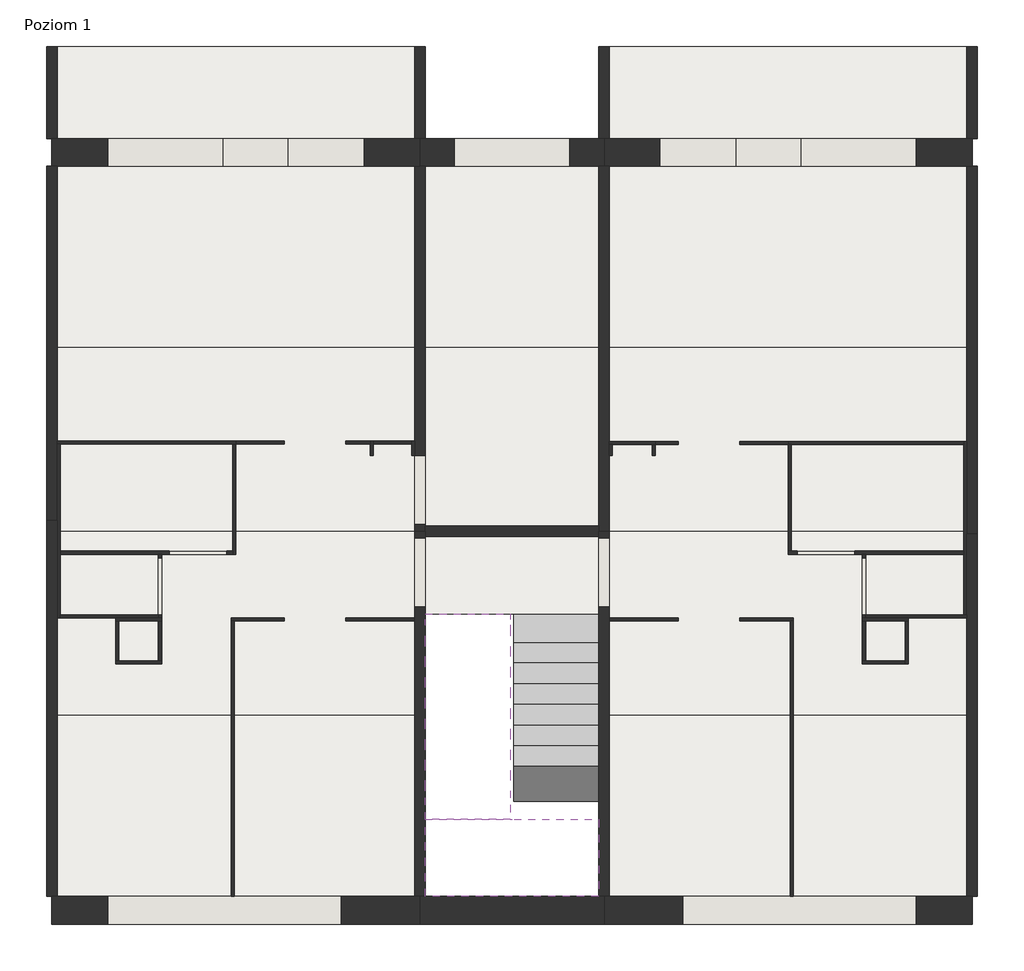
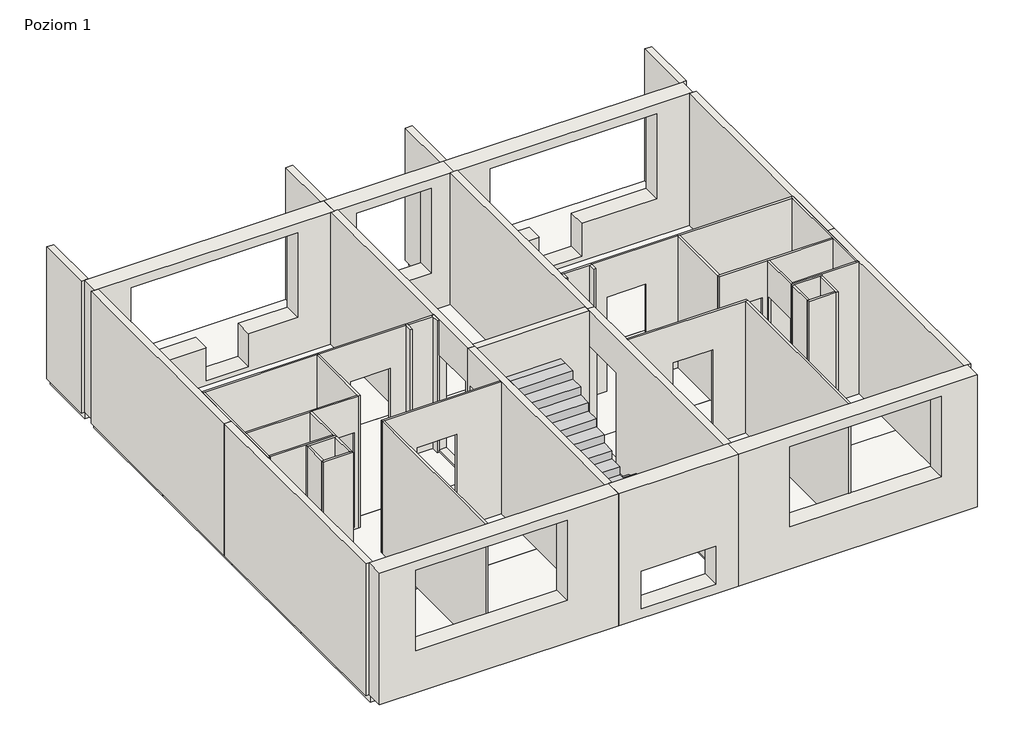
# One storey: 51 walls, 14 slabs, 2 proxies.
# Revit data of these elements (continued)
# Element 19 (IfcWall, "Prefab_ext_wall") (continued)
#   LastInspectionDate = 2025
#   MaintenanceInterval = 30
#   Phase Created = Etap 1
#   Base Constraint = Poziom 1
#   Top Constraint = Poziom 2
#   Materials on its faces: "Beton, wylewany na miejscu budowy"
# Element 20 (IfcWall, "Prefab_ext_wall")
#   CircularElementName = "Prefabricated Exterior Loadbearing Reinforced Concrete Wall"
#   CircularElementlDescription = "Medium conditions, damage in lower part"
#   CircularityNotes = "With exterior window opening"
#   Top Offset = 0 mm
#   Base Offset = 0 mm
#   wall height = 2800 mm
#   ExpectedServiceLife = 50
#   InstallationYear = 1973
#   LastInspectionDate = 2025
#   MaintenanceInterval = 30
#   Phase Created = Etap 1
#   Base Constraint = Poziom 1
#   Top Constraint = Poziom 2
#   Materials on its faces: "Beton, wylewany na miejscu budowy"
# Element 21 (IfcWall, "Prefab_ext_wall")
#   CircularElementName = "Prefabricated Exterior Loadbearing Reinforced Concrete Wall"
#   CircularElementlDescription = "Good condition"
#   CircularityNotes = "With exterior window opening"
#   Top Offset = 0 mm
#   Base Offset = 0 mm
#   wall height = 2800 mm
#   ExpectedServiceLife = 50
#   InstallationYear = 1973
#   MaintenanceInterval = 30
#   Phase Created = Etap 1
#   Base Constraint = Poziom 1
#   Top Constraint = Poziom 2
#   Materials on its faces: "Beton, wylewany na miejscu budowy"
# Element 22 (IfcWall, "Prefab_ext_wall")
#   CircularElementName = "Prefabricated Exterior Loadbearing Reinforced Concrete Wall"
#   CircularElementlDescription = "Bad condition"
#   CircularityNotes = "With exterior window opening"
#   Top Offset = 0 mm
#   Base Offset = 0 mm
#   wall height = 2800 mm
#   ExpectedServiceLife = 50
#   InstallationYear = 1973
#   MaintenanceInterval = 30
#   Phase Created = Etap 1
#   Base Constraint = Poziom 1
#   Top Constraint = Poziom 2
#   Materials on its faces: "Beton, wylewany na miejscu budowy"
# Element 23 (IfcWall, "Prefab_int_wall")
#   CircularElementName = "Prefabricated Reinforced Reinforced Concrete Bathroom Wall"
#   CircularElementlDescription = "The element looks to be in medium condition, mold present"
#   Top Offset = 0 mm
#   Base Offset = 0 mm
#   wall height = 2800 mm
#   ExpectedServiceLife = 50
#   InstallationYear = 1973
#   LastInspectionDate = 2025
#   MaintenanceInterval = 20
#   Phase Created = Etap 1
#   Base Constraint = Poziom 1
#   Top Constraint = Poziom 2
#   Materials on its faces: "Beton, wylewany na miejscu budowy"
# Elements 24, 26 (IfcWall, "Prefab_int_wall")
#   CircularElementName = "Prefabricated Reinforced Reinforced Concrete Interior Wall"
#   CircularElementlDescription = "Good condition, no major damage"
#   CircularityNotes = "With door opening"
#   Top Offset = 0 mm
#   Base Offset = 0 mm
#   wall height = 2800 mm
#   ExpectedServiceLife = 50
#   InstallationYear = 1973
#   LastInspectionDate = 2025
#   MaintenanceInterval = 40
#   Phase Created = Etap 1
#   Base Constraint = Poziom 1
#   Top Constraint = Poziom 2
#   Materials on its faces: "Beton, wylewany na miejscu budowy"
# Element 25 (IfcWall, "Prefab_int_wall")
#   CircularElementName = "Prefabricated Reinforced Reinforced Concrete Interior Wall"
#   CircularElementlDescription = "The element looks to be in good condition, no major damage"
#   Top Offset = 0 mm
#   Base Offset = 0 mm
#   wall height = 2800 mm
#   ExpectedServiceLife = 50
#   InstallationYear = 1973
#   LastInspectionDate = 2025
#   MaintenanceInterval = 40
#   Phase Created = Etap 1
#   Base Constraint = Poziom 1
#   Top Constraint = Poziom 2
#   Materials on its faces: "Beton, wylewany na miejscu budowy"
# Element 27 (IfcWall, "Prefab_int_wall")
#   CircularElementName = "Prefabricated Reinforced Reinforced Concrete Interior Wall"
#   CircularElementlDescription = "Good condition, minor dents and holes"
#   Top Offset = 0 mm
#   Base Offset = 0 mm
#   wall height = 2800 mm
#   ExpectedServiceLife = 50
#   InstallationYear = 1973
#   LastInspectionDate = 2025
#   MaintenanceInterval = 40
#   Phase Created = Etap 1
#   Base Constraint = Poziom 1
#   Top Constraint = Poziom 2
#   Materials on its faces: "Beton, wylewany na miejscu budowy"
# Elements 28, 30, 32 (IfcWall, "Prefab_int_wall")
#   CircularElementName = "Prefabricated Reinforced Reinforced Concrete Shaft Wall"
#   Top Offset = 0 mm
#   Base Offset = 0 mm
#   wall height = 2800 mm
#   ExpectedServiceLife = 50
#   InstallationYear = 1973
#   LastInspectionDate = 2004
#   MaintenanceInterval = 40
#   Phase Created = Etap 1
#   Base Constraint = Poziom 1
#   Top Constraint = Poziom 2
#   Materials on its faces: "Beton, wylewany na miejscu budowy"
# Element 29 (IfcWall, "Prefab_int_wall")
#   CircularElementName = "Prefabricated Reinforced Reinforced Concrete Shaft Wall"
#   CircularElementlDescription = "The element looks to be in good condition, no major damage"
#   Top Offset = 0 mm
#   Base Offset = 0 mm
#   wall height = 2800 mm
#   ExpectedServiceLife = 50
#   InstallationYear = 1973
#   LastInspectionDate = 2004
#   MaintenanceInterval = 40
#   Phase Created = Etap 1
#   Base Constraint = Poziom 1
#   Top Constraint = Poziom 2
#   Materials on its faces: "Beton, wylewany na miejscu budowy"
# Element 31 (IfcWall, "Prefab_int_wall")
#   CircularElementName = "Prefabricated Reinforced Reinforced Concrete Bathroom Wall"
#   CircularElementlDescription = "Good condition, no major damage"
#   CircularityNotes = "With door opening"
#   Top Offset = 0 mm
#   Base Offset = 0 mm
#   wall height = 2800 mm
#   ExpectedServiceLife = 50
#   InstallationYear = 1973
#   LastInspectionDate = 2004
#   MaintenanceInterval = 20
#   Phase Created = Etap 1
#   Base Constraint = Poziom 1
#   Top Constraint = Poziom 2
#   Materials on its faces: "Beton, wylewany na miejscu budowy"
# Element 33 (IfcWall, "Prefab_int_wall")
#   CircularElementName = "Prefabricated Reinforced Reinforced Concrete Bathroom Wall"
#   CircularElementlDescription = "The element looks to be in medium condition, mold present"
#   CircularityNotes = "With door opening"
#   Top Offset = 0 mm
#   Base Offset = 0 mm
#   wall height = 2800 mm
#   ExpectedServiceLife = 50
#   InstallationYear = 1973
#   LastInspectionDate = 2004
#   MaintenanceInterval = 20
#   Phase Created = Etap 1
#   Base Constraint = Poziom 1
#   Top Constraint = Poziom 2
#   Materials on its faces: "Beton, wylewany na miejscu budowy"
# Element 34 (IfcWall, "Prefab_int_wall")
#   CircularElementName = "Prefabricated Reinforced Reinforced Concrete Shaft Wall"
#   Top Offset = 0 mm
#   Base Offset = 0 mm
#   wall height = 2800 mm
#   ExpectedServiceLife = 50
#   InstallationYear = 1973
#   MaintenanceInterval = 40
#   Phase Created = Etap 1
#   Base Constraint = Poziom 1
#   Top Constraint = Poziom 2
#   Materials on its faces: "Beton, wylewany na miejscu budowy"
# Element 35 (IfcWall, "Prefab_int_wall")
#   CircularElementName = "Prefabricated Reinforced Reinforced Concrete Shaft Wall"
#   CircularElementlDescription = "The element looks to be in good condition, no major damage"
#   Top Offset = 0 mm
#   Base Offset = 0 mm
#   wall height = 2800 mm
#   ExpectedServiceLife = 50
#   InstallationYear = 1973
#   MaintenanceInterval = 40
#   Phase Created = Etap 1
#   Base Constraint = Poziom 1
#   Top Constraint = Poziom 2
#   Materials on its faces: "Beton, wylewany na miejscu budowy"
# Element 36 (IfcWall, "Prefab_int_wall")
#   CircularElementName = "Prefabricated Reinforced Reinforced Concrete Bathroom Wall"
#   CircularElementlDescription = "The element looks to be in good condition, no major damage"
#   Top Offset = 0 mm
#   Base Offset = 0 mm
#   wall height = 2800 mm
#   ExpectedServiceLife = 50
#   InstallationYear = 1973
#   Phase Created = Etap 1
#   Base Constraint = Poziom 1
#   Top Constraint = Poziom 2
#   Materials on its faces: "Beton, wylewany na miejscu budowy"
# Element 37 (IfcWall, "Prefab_int_wall")
#   CircularElementName = "Prefabricated Reinforced Reinforced Concrete Bathroom Wall"
#   CircularElementlDescription = "Good condition, no major damage"
#   CircularityNotes = "With door opening"
#   Top Offset = 0 mm
#   Base Offset = 0 mm
#   wall height = 2800 mm
#   InstallationYear = 1973
#   MaintenanceInterval = 20
#   Phase Created = Etap 1
#   Base Constraint = Poziom 1
#   Top Constraint = Poziom 2
#   Materials on its faces: "Beton, wylewany na miejscu budowy"
# Elements 38, 39 (IfcWall, "Prefab_int_wall")
#   CircularElementName = "Prefabricated Reinforced Reinforced Concrete Bathroom Wall"
#   Top Offset = 0 mm
#   Base Offset = 0 mm
#   wall height = 2800 mm
#   ExpectedServiceLife = 50
#   InstallationYear = 1973
#   MaintenanceInterval = 20
#   Phase Created = Etap 1
#   Base Constraint = Poziom 1
#   Top Constraint = Poziom 2
#   Materials on its faces: "Beton, wylewany na miejscu budowy"
# Element 40 (IfcWall, "Prefab_int_wall")
#   CircularElementName = "Prefabricated Reinforced Reinforced Concrete Bathroom Wall"
#   CircularityNotes = "With door opening"
#   Top Offset = 0 mm
#   Base Offset = 0 mm
#   wall height = 2800 mm
#   ExpectedServiceLife = 50
#   InstallationYear = 1973
#   MaintenanceInterval = 20
#   Phase Created = Etap 1
#   Base Constraint = Poziom 1
#   Top Constraint = Poziom 2
#   Materials on its faces: "Beton, wylewany na miejscu budowy"
# Element 41 (IfcWall, "Prefab_int_wall")
#   CircularElementName = "Prefabricated Reinforced Reinforced Concrete Bathroom Wall"
#   CircularElementlDescription = "Good condition, no major damage"
#   Top Offset = 0 mm
#   Base Offset = 0 mm
#   wall height = 2800 mm
#   ExpectedServiceLife = 50
#   InstallationYear = 1973
#   MaintenanceInterval = 20
#   Phase Created = Etap 1
#   Base Constraint = Poziom 1
#   Top Constraint = Poziom 2
#   Materials on its faces: "Beton, wylewany na miejscu budowy"
# Elements 42, 47 (IfcWall, "Prefab_int_wall")
#   CircularElementName = "Prefabricated Reinforced Reinforced Concrete Bathroom Wall"
#   Top Offset = 0 mm
#   Base Offset = 0 mm
#   wall height = 2800 mm
#   ExpectedServiceLife = 50
#   InstallationYear = 1973
#   LastInspectionDate = 2004
#   MaintenanceInterval = 20
#   Phase Created = Etap 1
#   Base Constraint = Poziom 1
#   Top Constraint = Poziom 2
#   Materials on its faces: "Beton, wylewany na miejscu budowy"
# Elements 43, 45, 49 (IfcWall, "Prefab_int_wall")
#   CircularElementName = "Prefabricated Reinforced Reinforced Concrete Interior Wall"
#   Top Offset = 0 mm
#   Base Offset = 0 mm
#   wall height = 2800 mm
#   ExpectedServiceLife = 50
#   InstallationYear = 1973
#   LastInspectionDate = 2004
#   MaintenanceInterval = 40
#   Phase Created = Etap 1
#   Base Constraint = Poziom 1
#   Top Constraint = Poziom 2
#   Materials on its faces: "Beton, wylewany na miejscu budowy"
# Element 44 (IfcWall, "Prefab_int_wall")
#   CircularElementName = "Prefabricated Reinforced Reinforced Concrete Interior Wall"
#   CircularElementlDescription = "Good condition, no major damage"
#   Top Offset = 0 mm
#   Base Offset = 0 mm
#   wall height = 2800 mm
#   ExpectedServiceLife = 50
#   InstallationYear = 1973
#   MaintenanceInterval = 40
#   Phase Created = Etap 1
#   Base Constraint = Poziom 1
#   Top Constraint = Poziom 2
#   Materials on its faces: "Beton, wylewany na miejscu budowy"
# Element 46 (IfcWall, "Prefab_int_wall")
#   CircularElementName = "Prefabricated Reinforced Reinforced Concrete Bathroom Wall"
#   CircularElementlDescription = "Medium condition"
#   Top Offset = 0 mm
#   Base Offset = 0 mm
#   wall height = 2800 mm
#   InstallationYear = 1973
#   MaintenanceInterval = 20
#   Phase Created = Etap 1
#   Base Constraint = Poziom 1
#   Top Constraint = Poziom 2
#   Materials on its faces: "Beton, wylewany na miejscu budowy"
# Element 48 (IfcWall, "Prefab_int_wall")
#   CircularElementName = "Prefabricated Reinforced Reinforced Concrete Interior Wall"
#   CircularElementlDescription = "Good condition, no major damage"
#   Top Offset = 0 mm
#   Base Offset = 0 mm
#   wall height = 2800 mm
#   ExpectedServiceLife = 50
#   InstallationYear = 1973
#   Phase Created = Etap 1
#   Base Constraint = Poziom 1
#   Top Constraint = Poziom 2
#   Materials on its faces: "Beton, wylewany na miejscu budowy"
# Element 50 (IfcWall, "Prefab_int_wall")
#   CircularElementName = "Prefabricated Reinforced Reinforced Concrete Interior Wall"
#   CircularityNotes = "With door opening"
#   Top Offset = 0 mm
#   Base Offset = 0 mm
#   wall height = 2800 mm
#   ExpectedServiceLife = 50
#   LastInspectionDate = 2025
#   MaintenanceInterval = 40
#   Phase Created = Etap 1
#   Base Constraint = Poziom 1
#   Top Constraint = Poziom 2
#   Materials on its faces: "Beton, wylewany na miejscu budowy"
# Element 51 (IfcWall, "Prefab_int_wall")
#   CircularElementName = "Prefabricated Reinforced Reinforced Concrete Shaft Wall"
#   CircularElementlDescription = "Good condition"
#   Top Offset = 0 mm
#   Base Offset = 0 mm
#   wall height = 2800 mm
#   ExpectedServiceLife = 50
#   InstallationYear = 1973
#   Phase Created = Etap 1
#   Base Constraint = Poziom 1
#   Top Constraint = Poziom 2
#   Materials on its faces: "Beton, wylewany na miejscu budowy"
# Element 52 (IfcWall, "Prefab_int_wall")
#   CircularElementName = "Prefabricated Reinforced Reinforced Concrete Interior Wall"
#   CircularElementlDescription = "Good condition"
#   CircularityNotes = "With door opening"
#   Top Offset = 0 mm
#   Base Offset = 0 mm
#   wall height = 2800 mm
#   ExpectedServiceLife = 50
#   InstallationYear = 1973
#   LastInspectionDate = 2025
#   MaintenanceInterval = 40
#   Phase Created = Etap 1
#   Base Constraint = Poziom 1
#   Top Constraint = Poziom 2
#   Materials on its faces: "Beton, wylewany na miejscu budowy"
# Element 53 (IfcWall, "Prefab_int_wall")
#   CircularElementName = "Prefabricated Loadbearing Reinforced Concrete Wall"
#   Top Offset = 0 mm
#   Base Offset = 0 mm
#   wall height = 2800 mm
#   ExpectedServiceLife = 50
#   InstallationYear = 1973
#   LastInspectionDate = 2025
#   MaintenanceInterval = 40
#   Phase Created = Etap 1
#   Base Constraint = Poziom 1
#   Top Constraint = Poziom 2
#   Materials on its faces: "Beton, wylewany na miejscu budowy"
# Element 54 (IfcWall, "Prefab_int_wall")
#   CircularElementName = "Prefabricated Reinforced Reinforced Concrete Shaft Wall"
#   Top Offset = 0 mm
#   Base Offset = 0 mm
#   wall height = 2800 mm
#   ExpectedServiceLife = 50
#   InstallationYear = 1973
#   LastInspectionDate = 2025
#   MaintenanceInterval = 40
#   Phase Created = Etap 1
#   Base Constraint = Poziom 1
#   Top Constraint = Poziom 2
#   Materials on its faces: "Beton, wylewany na miejscu budowy"
# Element 55 (IfcWall, "Prefab_wall")
#   CircularElementName = "Prefabricated Loadbearing Reinforced Concrete Wall"
#   CircularElementlDescription = "Good condition, no major damage"
#   CircularityNotes = ""
#   Top Offset = 0 mm
#   Base Offset = 0 mm
#   Unconnected Height = 2800 mm
#   wall height = 2800 mm
#   ExpectedServiceLife = 50
#   InstallationYear = 1973
#   LastInspectionDate = 2025
#   MaintenanceInterval = 40
#   Phase Created = Etap 1
#   Base Constraint = Poziom 1
#   Top Constraint = Poziom 2
#   Materials on its faces: "Beton, wylewany na miejscu budowy"
# Element 56 (IfcWall, "Prefab_wall")
#   CircularElementName = "Prefabricated Loadbearing Reinforced Concrete Wall"
#   CircularElementlDescription = "The element looks to be in good condition, no major damage"
#   Top Offset = 0 mm
#   Base Offset = 0 mm
#   wall height = 2800 mm
#   ExpectedServiceLife = 50
#   InstallationYear = 1973
#   LastInspectionDate = 2025
#   MaintenanceInterval = 40
#   Phase Created = Etap 1
#   Base Constraint = Poziom 1
#   Top Constraint = Poziom 2
#   Materials on its faces: "Beton, wylewany na miejscu budowy"
# Element 57 (IfcWall, "Prefab_wall")
#   CircularElementName = "Prefabricated Loadbearing Reinforced Concrete Wall"
#   CircularElementlDescription = ""
#   CircularityNotes = ""
#   Top Offset = 0 mm
#   Base Offset = 0 mm
#   Unconnected Height = 2800 mm
#   wall height = 2800 mm
#   ExpectedServiceLife = 50
#   InstallationYear = 1973
#   LastInspectionDate = 2025
#   MaintenanceInterval = 40
#   Phase Created = Etap 1
#   Base Constraint = Poziom 1
#   Top Constraint = Poziom 2
#   Materials on its faces: "Beton, wylewany na miejscu budowy"
# Element 58 (IfcWall, "Prefab_wall")
#   CircularElementName = "Prefabricated Loadbearing Reinforced Concrete Wall"
#   CircularElementlDescription = "Good condition, no major damage"
#   Top Offset = 0 mm
#   Base Offset = 0 mm
#   wall height = 2800 mm
#   ExpectedServiceLife = 50
#   InstallationYear = 1973
#   LastInspectionDate = 2004
#   MaintenanceInterval = 40
#   Phase Created = Etap 1
#   Base Constraint = Poziom 1
#   Top Constraint = Poziom 2
#   Materials on its faces: "Beton, wylewany na miejscu budowy"
# Element 59 (IfcWall, "Prefab_wall")
#   CircularElementName = "Prefabricated Loadbearing Reinforced Concrete Wall"
#   CircularElementlDescription = "Good condition, minor damage in the hallway"
#   CircularityNotes = "With door opening"
#   Top Offset = 0 mm
#   Base Offset = 0 mm
#   Unconnected Height = 2800 mm
#   wall height = 2800 mm
#   InstallationYear = 1973
#   LastInspectionDate = 2025
#   MaintenanceInterval = 40
#   Phase Created = Etap 1
#   Base Constraint = Poziom 1
#   Top Constraint = Poziom 2
#   Materials on its faces: "Beton, wylewany na miejscu budowy"
# Element 60 (IfcWall, "Prefab_wall")
#   CircularElementName = "Prefabricated Loadbearing Reinforced Concrete Wall"
#   CircularElementlDescription = "Good condition, no major damage"
#   CircularityNotes = "With door opening"
#   Top Offset = 0 mm
#   Base Offset = 0 mm
#   Unconnected Height = 2800 mm
#   wall height = 2800 mm
#   ExpectedServiceLife = 50
#   InstallationYear = 1973
#   LastInspectionDate = 2025
#   MaintenanceInterval = 40
#   Phase Created = Etap 1
#   Base Constraint = Poziom 1
#   Top Constraint = Poziom 2
#   Materials on its faces: "Beton, wylewany na miejscu budowy"
# Element 61 (IfcWall, "Prefab_wall")
#   CircularElementName = "Prefabricated Exterior Balcony Wall"
#   CircularElementlDescription = "Bad condition"
#   Top Offset = 0 mm
#   Base Offset = 0 mm
#   wall height = 2800 mm
#   ExpectedServiceLife = 50
#   InstallationYear = 2009
#   LastInspectionDate = 2009
#   MaintenanceInterval = 30
#   Phase Created = Etap 1
#   Base Constraint = Poziom 1
#   Top Constraint = Poziom 2
#   Materials on its faces: "Beton, wylewany na miejscu budowy"
# Element 62 (IfcWall, "Prefab_wall")
#   CircularElementName = "Prefabricated Exterior Balcony Wall"
#   CircularElementlDescription = "Medium condition"
#   Top Offset = 0 mm
#   Base Offset = 0 mm
#   wall height = 2800 mm
#   ExpectedServiceLife = 50
#   InstallationYear = 2009
#   LastInspectionDate = 2009
#   Phase Created = Etap 1
#   Base Constraint = Poziom 1
#   Top Constraint = Poziom 2
#   Materials on its faces: "Beton, wylewany na miejscu budowy"
# Element 63 (IfcWall, "Prefab_wall")
#   CircularElementName = "Prefabricated Exterior Balcony Wall"
#   CircularElementlDescription = "Medium condition"
#   Top Offset = 0 mm
#   Base Offset = 0 mm
#   wall height = 2800 mm
#   ExpectedServiceLife = 50
#   InstallationYear = 1973
#   MaintenanceInterval = 30
#   Phase Created = Etap 1
#   Base Constraint = Poziom 1
#   Top Constraint = Poziom 2
#   Materials on its faces: "Beton, wylewany na miejscu budowy"
# Element 64 (IfcWall, "Prefab_wall")
#   CircularElementName = "Prefabricated Exterior Balcony Wall"
#   CircularElementlDescription = "Medium condition, damage in lower part"
#   Top Offset = 0 mm
#   Base Offset = 0 mm
#   wall height = 2800 mm
#   ExpectedServiceLife = 50
#   InstallationYear = 1973
#   MaintenanceInterval = 30
#   Phase Created = Etap 1
#   Base Constraint = Poziom 1
#   Top Constraint = Poziom 2
#   Materials on its faces: "Beton, wylewany na miejscu budowy"
# Element 65 (IfcWall, "Prefab_wall")
#   CircularElementName = "Prefabricated Loadbearing Reinforced Concrete Wall"
#   Top Offset = 0 mm
#   Base Offset = 0 mm
#   wall height = 2800 mm
#   ExpectedServiceLife = 50
#   InstallationYear = 1973
#   MaintenanceInterval = 40
#   Phase Created = Etap 1
#   Base Constraint = Poziom 1
#   Top Constraint = Poziom 2
#   Materials on its faces: "Beton, wylewany na miejscu budowy"
# Element 66 (IfcWall, "Prefab_wall")
#   CircularElementName = "Prefabricated Loadbearing Reinforced Concrete Wall"
#   CircularElementlDescription = "Good condition"
#   CircularityNotes = "With door opening"
#   Top Offset = 0 mm
#   Base Offset = 0 mm
#   Unconnected Height = 2800 mm
#   wall height = 2800 mm
#   ExpectedServiceLife = 50
#   InstallationYear = 1973
#   LastInspectionDate = 2025
#   MaintenanceInterval = 40
#   Phase Created = Etap 1
#   Base Constraint = Poziom 1
#   Top Constraint = Poziom 2
#   Materials on its faces: "Beton, wylewany na miejscu budowy"
# Element 67 (IfcWall, "Prefab_wall")
#   CircularElementName = "Prefabricated Loadbearing Reinforced Concrete Wall"
#   CircularElementlDescription = "Good condition"
#   CircularityNotes = ""
#   Top Offset = 0 mm
#   Base Offset = 0 mm
#   Unconnected Height = 2800 mm
#   wall height = 2800 mm
#   ExpectedServiceLife = 50
#   LastInspectionDate = 2025
#   MaintenanceInterval = 40
#   Phase Created = Etap 1
#   Base Constraint = Poziom 1
#   Top Constraint = Poziom 2
#   Materials on its faces: "Beton, wylewany na miejscu budowy"
# Materials
#   "Beton, wylewany na miejscu budowy": class "Beton", colour RGB 192 192 192, transparency 0, Description = "materiał fizyczny", Cost = 0
